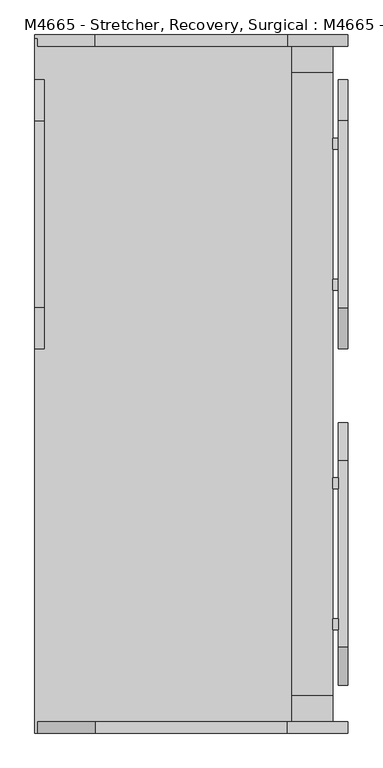
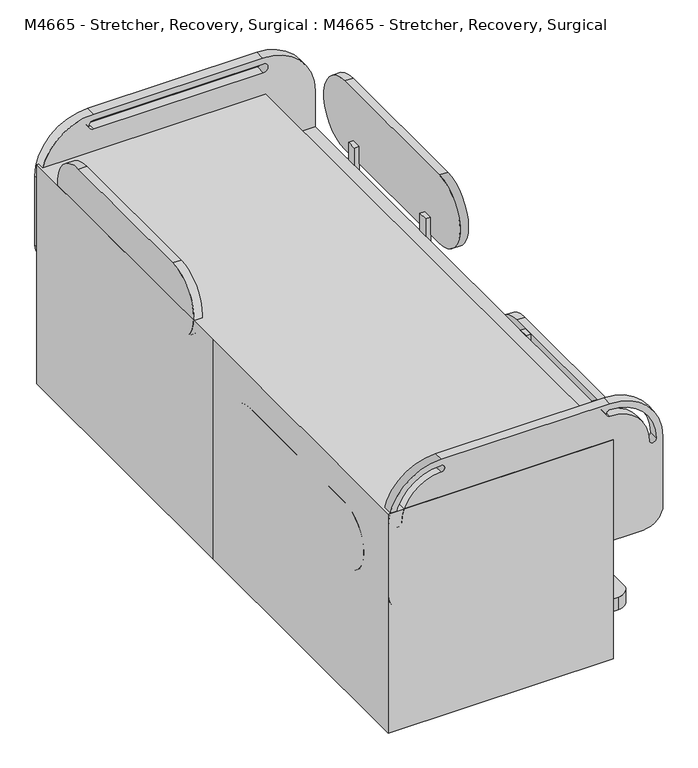
"""IFC4 building model written with IfcOpenShell, lengths in millimetres: proxy geometry, M4665 - Stretcher, Recovery, Surgical : M4665 - Stretcher, Recovery, Surgical."""

import ifcopenshell
import ifcopenshell.guid

model = None  # the IFC model being written
_history = None  # IfcOwnerHistory: only IFC2X3 demands one
_inside = {}  # id of a spatial element -> (the spatial element, [elements in it])
_under = {}  # id of a project, library or spatial element -> (it, [spatial elements below it])
_declared = {}  # id of a project -> (the project, [libraries it declares])
_typed = {}  # id of a type object -> (the type object, [elements of that type])
_made_of = {}  # id of a material, layer set ... -> (it, [elements and type objects made of it])


def new_model(schema):
    """Start an empty IFC model of exactly this schema.

    Asked for "IFC4X3", IfcOpenShell would pick the latest addendum, in which some entities
    have other attributes; the version numbers below select the first issue.
    IFC2X3 requires an IfcOwnerHistory on every rooted entity: one is made here for all.
    """
    global model, _history
    if schema == "IFC4X3":
        model = ifcopenshell.file(schema_version=(4, 3, 0, 0))
    else:
        model = ifcopenshell.file(schema=schema)
    _inside.clear()
    _under.clear()
    _declared.clear()
    _typed.clear()
    _made_of.clear()
    _history = None
    if model.schema == "IFC2X3":
        org = make("IfcOrganization", Name="unknown")
        user = make(
            "IfcPersonAndOrganization",
            ThePerson=make("IfcPerson", FamilyName="unknown"),
            TheOrganization=org,
        )
        app = make(
            "IfcApplication",
            ApplicationDeveloper=org,
            Version="unknown",
            ApplicationFullName="unknown",
            ApplicationIdentifier="unknown",
        )
        _history = make(
            "IfcOwnerHistory",
            OwningUser=user,
            OwningApplication=app,
            ChangeAction="ADDED",
            CreationDate=0,
        )
    return model


def make(cls, **values):
    """One entity of the class cls with the attributes given. An attribute that is None is left unset."""
    return model.create_entity(
        cls, **{name: value for name, value in values.items() if value is not None}
    )


def rooted(cls, **values):
    """An entity with a GlobalId (a new one), such as an element, a storey or a relation."""
    return make(cls, GlobalId=ifcopenshell.guid.new(), OwnerHistory=_history, **values)


def si_unit(unit_type, name, prefix=None):
    """IfcSIUnit, for example si_unit("LENGTHUNIT", "METRE", prefix="MILLI")."""
    return make("IfcSIUnit", UnitType=unit_type, Prefix=prefix, Name=name)


def assignment(units):
    """IfcUnitAssignment: the units of a project."""
    return None if units is None else make("IfcUnitAssignment", Units=units)


def point(xyz):
    """IfcCartesianPoint."""
    return None if xyz is None else make("IfcCartesianPoint", Coordinates=xyz)


def direction(xyz):
    """IfcDirection."""
    return None if xyz is None else make("IfcDirection", DirectionRatios=xyz)


def frame(location, z_axis=None, x_axis=None):
    """IfcAxis2Placement3D, a coordinate frame: its origin and axes. An axis left out is left unset."""
    return make(
        "IfcAxis2Placement3D",
        Location=point(location),
        Axis=direction(z_axis),
        RefDirection=direction(x_axis),
    )


def frame_2d(location, x_axis=None):
    """IfcAxis2Placement2D, a coordinate frame in the plane: its origin and x axis."""
    return make(
        "IfcAxis2Placement2D", Location=point(location), RefDirection=direction(x_axis)
    )


def origin():
    """The frame at (0, 0, 0) with its axes left unset."""
    return frame((0.0, 0.0, 0.0))


def place(relative_to, where):
    """IfcLocalPlacement: puts the frame where relative to a parent placement (None: the world)."""
    return make(
        "IfcLocalPlacement", PlacementRelTo=relative_to, RelativePlacement=where
    )


def context(
    kind, dimensions, precision=None, world=None, true_north=None, identifier=None
):
    """IfcGeometricRepresentationContext, for example the 3D "Model" context."""
    return make(
        "IfcGeometricRepresentationContext",
        ContextIdentifier=identifier,
        ContextType=kind,
        CoordinateSpaceDimension=dimensions,
        Precision=precision,
        WorldCoordinateSystem=world,
        TrueNorth=true_north,
    )


def project(units=None, contexts=None):
    """IfcProject with its units and contexts."""
    return rooted(
        "IfcProject",
        Name="project",
        RepresentationContexts=contexts,
        UnitsInContext=assignment(units),
    )


def spatial(cls, under=None, at=None, **own):
    """A site, building, storey or space (cls), placed at a placement, below another one or the project."""
    s = rooted(cls, ObjectPlacement=at, **own)
    if under is not None:
        _under.setdefault(under.id(), (under, []))[1].append(s)
    return s


def polyline(points):
    """IfcPolyline through the points."""
    return make("IfcPolyline", Points=[point(p) for p in points])


def circle_curve(where, radius):
    """IfcCircle in the frame where."""
    return make("IfcCircle", Position=where, Radius=radius)


def trimmed(basis, trim1, trim2, sense, master):
    """IfcTrimmedCurve: the piece of a basis curve between two trims."""
    return make(
        "IfcTrimmedCurve",
        BasisCurve=basis,
        Trim1=trim1,
        Trim2=trim2,
        SenseAgreement=sense,
        MasterRepresentation=master,
    )


def segment(curve, same_sense, transition):
    """IfcCompositeCurveSegment."""
    return make(
        "IfcCompositeCurveSegment",
        Transition=transition,
        SameSense=same_sense,
        ParentCurve=curve,
    )


def composite_curve(segments, self_intersect=None):
    """IfcCompositeCurve: segments joined end to end."""
    return make("IfcCompositeCurve", Segments=segments, SelfIntersect=self_intersect)


def outline(outer, holes=None, kind="AREA"):
    """IfcArbitraryClosedProfileDef: a profile drawn as a closed curve; with holes, ...WithVoids."""
    if holes is None:
        return make("IfcArbitraryClosedProfileDef", ProfileType=kind, OuterCurve=outer)
    return make(
        "IfcArbitraryProfileDefWithVoids",
        ProfileType=kind,
        OuterCurve=outer,
        InnerCurves=holes,
    )


def extrude(swept, where, along, depth):
    """IfcExtrudedAreaSolid: the profile swept, set in the frame where, extruded along a direction by depth."""
    return make(
        "IfcExtrudedAreaSolid",
        SweptArea=swept,
        Position=where,
        ExtrudedDirection=direction(along),
        Depth=depth,
    )


def faces_of(points, faces, orient=None, outer=None):
    """IfcFace entities. A face is a list of loops; a loop is a list of indices into points, from 0.

    orient and outer hold one flag for each loop. By default every Orientation is true, the
    first loop of a face is its IfcFaceOuterBound and the others are IfcFaceBound.
    """
    made = []
    for i, loops in enumerate(faces):
        bounds = []
        for j, loop in enumerate(loops):
            is_outer = j == 0 if outer is None else outer[i][j]
            bounds.append(
                make(
                    "IfcFaceOuterBound" if is_outer else "IfcFaceBound",
                    Bound=make("IfcPolyLoop", Polygon=[points[k] for k in loop]),
                    Orientation=True if orient is None else orient[i][j],
                )
            )
        made.append(make("IfcFace", Bounds=bounds))
    return made


def faceted_brep(points, faces, orient=None, outer=None, voids=None):
    """IfcFacetedBrep: a solid bounded by flat faces; with voids (closed shells), ...WithVoids."""
    shared = [point(p) for p in points]
    hull = make("IfcClosedShell", CfsFaces=faces_of(shared, faces, orient, outer))
    if voids is None:
        return make("IfcFacetedBrep", Outer=hull)
    return make(
        "IfcFacetedBrepWithVoids",
        Outer=hull,
        Voids=[
            make(cls, CfsFaces=faces_of(shared, fs, o, b)) for cls, fs, o, b in voids
        ],
    )


def shape(context_of_items, identifier, shape_type, items):
    """IfcShapeRepresentation: the items that make up one representation, for example the "Body"."""
    return make(
        "IfcShapeRepresentation",
        ContextOfItems=context_of_items,
        RepresentationIdentifier=identifier,
        RepresentationType=shape_type,
        Items=items,
    )


def source(mapping_origin, context_of_items, identifier, shape_type, items):
    """IfcRepresentationMap: a shape defined once, which mapped items show again and again."""
    return make(
        "IfcRepresentationMap",
        MappingOrigin=mapping_origin,
        MappedRepresentation=shape(context_of_items, identifier, shape_type, items),
    )


def transform(
    local_origin,
    x_axis=None,
    y_axis=None,
    z_axis=None,
    scale=None,
    scale2=None,
    scale3=None,
    uniform=True,
):
    """IfcCartesianTransformationOperator3D, or its non-uniform kind. x_axis, y_axis, z_axis: its Axis1, 2, 3."""
    if uniform:
        return make(
            "IfcCartesianTransformationOperator3D",
            Axis1=direction(x_axis),
            Axis2=direction(y_axis),
            LocalOrigin=point(local_origin),
            Scale=scale,
            Axis3=direction(z_axis),
        )
    return make(
        "IfcCartesianTransformationOperator3DnonUniform",
        Axis1=direction(x_axis),
        Axis2=direction(y_axis),
        LocalOrigin=point(local_origin),
        Scale=scale,
        Axis3=direction(z_axis),
        Scale2=scale2,
        Scale3=scale3,
    )


def mapped(mapping_source, mapping_target):
    """IfcMappedItem: shows the shape of a source again, moved by a transform."""
    return make(
        "IfcMappedItem", MappingSource=mapping_source, MappingTarget=mapping_target
    )


def made_of(thing, what):
    """Note that an element or type object is made of a material, layer set ...; save() writes the relation."""
    if what is not None:
        _made_of.setdefault(what.id(), (what, []))[1].append(thing)
    return thing


def element(
    cls,
    number,
    at=None,
    inside=None,
    cuts=None,
    type_object=None,
    material=None,
    context=None,
    identifier="Body",
    shape_type=None,
    held_by="IfcProductDefinitionShape",
    body=None,
    shapes=None,
    **own,
):
    """One element of the class cls, such as IfcWall. Its Tag is "e" and its number.

    at: its placement. inside: the storey or other place that contains it. cuts: it is an
    opening in that element (IfcRelVoidsElement). A single representation is given by context,
    identifier, shape_type and body (its items); several are given by shapes. held_by: the class
    of the entity that holds the representations. save() writes the other relations.
    """
    e = rooted(cls, Tag="e%d" % number, ObjectPlacement=at, **own)
    if body is not None:
        shapes = [shape(context, identifier, shape_type, body)]
    if shapes is not None:
        e.Representation = make(held_by, Representations=shapes)
    if inside is not None:
        _inside.setdefault(inside.id(), (inside, []))[1].append(e)
    if cuts is not None:
        rooted(
            "IfcRelVoidsElement", RelatingBuildingElement=cuts, RelatedOpeningElement=e
        )
    if type_object is not None:
        _typed.setdefault(type_object.id(), (type_object, []))[1].append(e)
    return made_of(e, material)


def aggregate(whole, parts):
    """IfcRelAggregates: a whole, such as a stair, and the parts it consists of."""
    return rooted("IfcRelAggregates", RelatingObject=whole, RelatedObjects=parts)


def save(model, path):
    """Write the relations noted so far, then the file.

    IfcRelAggregates (storeys below a building ...), IfcRelContainedInSpatialStructure (elements
    in a storey), IfcRelDefinesByType, IfcRelAssociatesMaterial and IfcRelDeclares: one each for
    every whole, place, type object, material and project.
    """
    for whole, parts in _under.values():
        aggregate(whole, parts)
    for where, things in _inside.values():
        rooted(
            "IfcRelContainedInSpatialStructure",
            RelatedElements=things,
            RelatingStructure=where,
        )
    for kind, things in _typed.values():
        rooted("IfcRelDefinesByType", RelatedObjects=things, RelatingType=kind)
    for what, things in _made_of.values():
        rooted("IfcRelAssociatesMaterial", RelatedObjects=things, RelatingMaterial=what)
    for by, libraries in _declared.values():
        rooted("IfcRelDeclares", RelatingContext=by, RelatedDefinitions=libraries)
    model.write(path)


def plane_surface(at):
    """IfcPlane: the flat surface through the origin of the frame at, square to its z axis."""
    return make("IfcPlane", Position=at)


def cylinder_surface(at, radius):
    """IfcCylindricalSurface: all points at the distance radius from the z axis of the frame at."""
    return make("IfcCylindricalSurface", Position=at, Radius=radius)


def revolved_surface(curve, axis_point, axis_direction):
    """IfcSurfaceOfRevolution: the curve turned about the line through axis_point along axis_direction."""
    return make(
        "IfcSurfaceOfRevolution",
        SweptCurve=make("IfcArbitraryOpenProfileDef", ProfileType="CURVE", Curve=curve),
        AxisPosition=make("IfcAxis1Placement", Location=point(axis_point), Axis=direction(axis_direction)),
    )


def advanced_brep(points, edges, surfaces, faces):
    """IfcAdvancedBrep: a solid bounded by faces that lie on surfaces and meet in shared edges.

    An edge is (start, end): straight between two places in points (the first is 0);
    or (start, end, curve); or (start, end, curve, False) where it runs against its curve.
    A face is (place in surfaces, loops), or (place, loops, False) where it looks against
    its surface's normal. A loop lists edges by number (the first is 1), with a minus sign
    where the edge is run from its end to its start. The first loop is the outer one.
    """
    corners = [point(p) for p in points]
    vertices = [make("IfcVertexPoint", VertexGeometry=c) for c in corners]
    made = []
    for start, end, *more in edges:
        made.append(
            make(
                "IfcEdgeCurve",
                EdgeStart=vertices[start],
                EdgeEnd=vertices[end],
                EdgeGeometry=more[0] if more else make("IfcPolyline", Points=[corners[start], corners[end]]),
                SameSense=more[1] if len(more) > 1 else True,
            )
        )
    hull = []
    for where, loops, *sense in faces:
        bounds = []
        for j, loop in enumerate(loops):
            ring = [make("IfcOrientedEdge", EdgeElement=made[abs(k) - 1], Orientation=k > 0) for k in loop]
            bounds.append(
                make(
                    "IfcFaceOuterBound" if j == 0 else "IfcFaceBound",
                    Bound=make("IfcEdgeLoop", EdgeList=ring),
                    Orientation=True,
                )
            )
        hull.append(make("IfcAdvancedFace", Bounds=bounds, FaceSurface=surfaces[where], SameSense=sense[0] if sense else True))
    return make("IfcAdvancedBrep", Outer=make("IfcClosedShell", CfsFaces=hull))


def m4665_stretcher_recovery_surgical_m4665_stretcher_recovery_9e5d2991(model_context):
    return source(origin(), model_context, "Body", "SolidModel", [
        extrude(outline(composite_curve([segment(trimmed(circle_curve(frame_2d((977.7599321, 51.5042315)), 51.5042315), [point((926.2557006, 51.5042315))], [point((1029.2641636, 51.5042315))], False, "CARTESIAN"), True, "CONTINUOUS"), segment(trimmed(circle_curve(frame_2d((977.7599321, 51.5042315)), 51.5042315), [point((1029.2641636, 51.5042315))], [point((926.2557006, 51.5042315))], False, "CARTESIAN"), True, "CONTINUOUS")], self_intersect=False)), frame((-292.1, 0.0, 0.0), z_axis=(1.0, 0.0, 0.0), x_axis=(0.0, 1.0, 0.0)), (0.0, 0.0, 1.0), 25.4),
        extrude(outline(composite_curve([segment(trimmed(circle_curve(frame_2d((977.7599321, 51.5042315)), 51.5042315), [point((926.2557006, 51.5042315))], [point((1029.2641636, 51.5042315))], False, "CARTESIAN"), True, "CONTINUOUS"), segment(trimmed(circle_curve(frame_2d((977.7599321, 51.5042315)), 51.5042315), [point((1029.2641636, 51.5042315))], [point((926.2557006, 51.5042315))], False, "CARTESIAN"), True, "CONTINUOUS")], self_intersect=False)), frame((457.2, 0.0, 0.0), z_axis=(1.0, 0.0, 0.0), x_axis=(0.0, 1.0, 0.0)), (0.0, 0.0, 1.0), 25.4),
        extrude(outline(composite_curve([segment(trimmed(circle_curve(frame_2d((-965.0599321, 51.5042315)), 51.5042315), [point((-913.5557006, 51.5042315))], [point((-1016.5641636, 51.5042315))], False, "CARTESIAN"), True, "CONTINUOUS"), segment(trimmed(circle_curve(frame_2d((-965.0599321, 51.5042315)), 51.5042315), [point((-1016.5641636, 51.5042315))], [point((-913.5557006, 51.5042315))], False, "CARTESIAN"), True, "CONTINUOUS")], self_intersect=False)), frame((457.2, 0.0, 0.0), z_axis=(1.0, 0.0, 0.0), x_axis=(0.0, 1.0, 0.0)), (0.0, 0.0, 1.0), 25.4),
        advanced_brep(
        [(450.85, 990.3863453, 60.4258647), (450.85, 985.39125, 48.3666377), (450.85, 966.5580857, 50.8460708), (450.85, 966.5580857, 108.9715457), (450.85, 976.2356274, 130.175), (450.85, 1006.5868486, 130.175), (450.85, 1014.4209258, 118.4504749), (488.95, 990.3863453, 60.4258647), (488.95, 1014.4209258, 118.4504749), (488.95, 1006.5868486, 130.175), (488.95, 976.2356274, 130.175), (488.95, 966.5580857, 108.9715457), (488.95, 966.5580857, 50.8460708), (488.95, 985.39125, 48.3666377), (457.0636195, 1014.4209258, 118.4504749), (457.0636195, 990.3863453, 60.4258647), (482.4636195, 990.3863453, 60.4258647), (482.4636195, 1014.4209258, 118.4504749), (482.4636195, 1014.7946321, 123.825), (457.0636195, 1014.7946321, 123.825), (457.0636195, 966.5580857, 108.9715457), (457.0636195, 973.337402, 123.825), (482.4636195, 973.337402, 123.825), (482.4636195, 966.5580857, 108.9715457), (457.0636195, 966.5580857, 50.8460708), (482.4636195, 966.5580857, 50.8460708), (457.0636195, 985.39125, 48.3666377), (482.4636195, 985.39125, 48.3666377)],
        [
            (0, 1),
            (1, 2, circle_curve(frame((450.85, 976.1378796, 50.8460708), z_axis=(-1.0, 0.0, 0.0), x_axis=(0.0, -1.0, 0.0)), 9.5797939)),
            (2, 3),
            (3, 4),
            (4, 5),
            (5, 6, circle_curve(frame((450.85, 1006.5868486, 121.6954559), z_axis=(-1.0, 0.0, 0.0), x_axis=(0.0, -1.0, 0.0)), 8.4795441)),
            (6, 0),
            (7, 8),
            (8, 9, circle_curve(frame((488.95, 1006.5868486, 121.6954559), z_axis=(1.0, 0.0, 0.0), x_axis=(0.0, -1.0, 0.0)), 8.4795441)),
            (9, 10),
            (10, 11),
            (11, 12),
            (12, 13, circle_curve(frame((488.95, 976.1378796, 50.8460708), z_axis=(1.0, 0.0, 0.0), x_axis=(0.0, -1.0, 0.0)), 9.5797939)),
            (13, 7),
            (6, 14),
            (14, 15),
            (15, 0),
            (7, 16),
            (16, 17),
            (17, 8),
            (5, 9),
            (17, 18, circle_curve(frame((482.4636195, 1006.5868486, 121.6954559), z_axis=(1.0, 0.0, 0.0), x_axis=(0.0, -1.0, 0.0)), 8.4795441)),
            (18, 19),
            (19, 14, circle_curve(frame((457.0636195, 1006.5868486, 121.6954559), z_axis=(-1.0, 0.0, 0.0), x_axis=(0.0, -1.0, 0.0)), 8.4795441)),
            (4, 10),
            (3, 20),
            (20, 21),
            (21, 22),
            (22, 23),
            (23, 11),
            (2, 24),
            (24, 20),
            (23, 25),
            (25, 12),
            (1, 26),
            (26, 24, circle_curve(frame((457.0636195, 976.1378796, 50.8460708), z_axis=(-1.0, 0.0, 0.0), x_axis=(0.0, -1.0, 0.0)), 9.5797939)),
            (25, 27, circle_curve(frame((482.4636195, 976.1378796, 50.8460708), z_axis=(1.0, 0.0, 0.0), x_axis=(0.0, -1.0, 0.0)), 9.5797939)),
            (27, 13),
            (15, 26),
            (27, 16),
            (18, 22),
            (21, 19),
        ],
        [
            plane_surface(frame((450.85, 990.3863453, 60.4258647), z_axis=(-1.0, 0.0, 0.0), x_axis=(0.0, -0.3826834323651177, -0.9238795325112752))),
            plane_surface(frame((488.95, 990.3863453, 60.4258647), z_axis=(1.0, 0.0, 0.0), x_axis=(0.0, 0.3826834323651177, 0.9238795325112752))),
            plane_surface(frame((450.85, 1014.4209258, 118.4504749), z_axis=(0.0, 0.9238795325112839, -0.38268343236509705), x_axis=(1.0, 0.0, 0.0))),
            cylinder_surface(frame((488.95, 1006.5868486, 121.6954559), z_axis=(-1.0, 0.0, 0.0), x_axis=(0.0, -1.0, 0.0)), 8.4795441),
            plane_surface(frame((450.85, 976.2356274, 130.175), z_axis=(0.0, 0.0, 1.0), x_axis=(1.0, 0.0, 0.0))),
            plane_surface(frame((450.85, 966.5580857, 108.9715457), z_axis=(0.0, -0.9097252183510659, 0.4152108224698697), x_axis=(1.0, 0.0, 0.0))),
            plane_surface(frame((450.85, 966.5580857, 50.8460708), z_axis=(0.0, -1.0, 0.0), x_axis=(1.0, 0.0, 0.0))),
            cylinder_surface(frame((488.95, 976.1378796, 50.8460708), z_axis=(-1.0, 0.0, 0.0), x_axis=(0.0, -1.0, 0.0)), 9.5797939),
            plane_surface(frame((450.85, 990.3863453, 60.4258647), z_axis=(0.0, 0.9238795325112752, -0.3826834323651177), x_axis=(1.0, 0.0, 0.0))),
            plane_surface(frame((482.4636195, 889.3256309, 123.825), z_axis=(0.0, 0.0, -1.0), x_axis=(0.0, 1.0, 0.0))),
            plane_surface(frame((482.4636195, 889.3256309, 0.0), z_axis=(-1.0, 0.0, 0.0), x_axis=(0.0, 1.0, 0.0))),
            plane_surface(frame((457.0636195, 889.3256309, 123.825), z_axis=(1.0, 0.0, 0.0), x_axis=(0.0, 1.0, 0.0))),
        ],
        [
            (0, [[1, 2, 3, 4, 5, 6, 7]]),
            (1, [[8, 9, 10, 11, 12, 13, 14]]),
            (2, [[-7, 15, 16, 17]]),
            (2, [[-8, 18, 19, 20]]),
            (3, [[-6, 21, -9, -20, 22, 23, 24, -15]]),
            (4, [[-5, 25, -10, -21]]),
            (5, [[-4, 26, 27, 28, 29, 30, -11, -25]]),
            (6, [[-3, 31, 32, -26]]),
            (6, [[-12, -30, 33, 34]]),
            (7, [[-2, 35, 36, -31]]),
            (7, [[-13, -34, 37, 38]]),
            (8, [[-1, -17, 39, -35]]),
            (8, [[-14, -38, 40, -18]]),
            (9, [[41, -28, 42, -23]]),
            (10, [[-41, -22, -19, -40, -37, -33, -29]]),
            (11, [[-42, -27, -32, -36, -39, -16, -24]]),
        ],
    ),
        advanced_brep(
        [(-266.5636195, 973.337402, 123.825), (-266.5636195, 1014.7946321, 123.825), (-266.5636195, 1014.4209258, 118.4504749), (-266.5636195, 990.3863453, 60.4258647), (-266.5636195, 985.39125, 48.3666377), (-266.5636195, 966.5580857, 50.8460708), (-266.5636195, 966.5580857, 108.9715457), (-291.9636195, 1014.7946321, 123.825), (-291.9636195, 973.337402, 123.825), (-291.9636195, 966.5580857, 108.9715457), (-291.9636195, 966.5580857, 50.8460708), (-291.9636195, 985.39125, 48.3666377), (-291.9636195, 990.3863453, 60.4258647), (-291.9636195, 1014.4209258, 118.4504749), (-260.35, 990.3863453, 60.4258647), (-260.35, 1014.4209258, 118.4504749), (-260.35, 1006.5868486, 130.175), (-260.35, 976.2356274, 130.175), (-260.35, 966.5580857, 108.9715457), (-260.35, 966.5580857, 50.8460708), (-260.35, 985.39125, 48.3666377), (-298.45, 990.3863453, 60.4258647), (-298.45, 985.39125, 48.3666377), (-298.45, 966.5580857, 50.8460708), (-298.45, 966.5580857, 108.9715457), (-298.45, 976.2356274, 130.175), (-298.45, 1006.5868486, 130.175), (-298.45, 1014.4209258, 118.4504749)],
        [
            (0, 1),
            (1, 2, circle_curve(frame((-266.5636195, 1006.5868486, 121.6954559), z_axis=(-1.0, 0.0, 0.0), x_axis=(0.0, -1.0, 0.0)), 8.4795441)),
            (2, 3),
            (3, 4),
            (4, 5, circle_curve(frame((-266.5636195, 976.1378796, 50.8460708), z_axis=(-1.0, 0.0, 0.0), x_axis=(0.0, -1.0, 0.0)), 9.5797939)),
            (5, 6),
            (6, 0),
            (7, 8),
            (8, 9),
            (9, 10),
            (10, 11, circle_curve(frame((-291.9636195, 976.1378796, 50.8460708), z_axis=(1.0, 0.0, 0.0), x_axis=(0.0, -1.0, 0.0)), 9.5797939)),
            (11, 12),
            (12, 13),
            (13, 7, circle_curve(frame((-291.9636195, 1006.5868486, 121.6954559), z_axis=(1.0, 0.0, 0.0), x_axis=(0.0, -1.0, 0.0)), 8.4795441)),
            (7, 1),
            (0, 8),
            (14, 15),
            (15, 16, circle_curve(frame((-260.35, 1006.5868486, 121.6954559), z_axis=(1.0, 0.0, 0.0), x_axis=(0.0, -1.0, 0.0)), 8.4795441)),
            (16, 17),
            (17, 18),
            (18, 19),
            (19, 20, circle_curve(frame((-260.35, 976.1378796, 50.8460708), z_axis=(1.0, 0.0, 0.0), x_axis=(0.0, -1.0, 0.0)), 9.5797939)),
            (20, 14),
            (21, 22),
            (22, 23, circle_curve(frame((-298.45, 976.1378796, 50.8460708), z_axis=(-1.0, 0.0, 0.0), x_axis=(0.0, -1.0, 0.0)), 9.5797939)),
            (23, 24),
            (24, 25),
            (25, 26),
            (26, 27, circle_curve(frame((-298.45, 1006.5868486, 121.6954559), z_axis=(-1.0, 0.0, 0.0), x_axis=(0.0, -1.0, 0.0)), 8.4795441)),
            (27, 21),
            (20, 4),
            (3, 14),
            (21, 12),
            (11, 22),
            (19, 5),
            (10, 23),
            (18, 6),
            (9, 24),
            (17, 25),
            (16, 26),
            (15, 2),
            (13, 27),
        ],
        [
            plane_surface(frame((-266.5636195, 889.3256309, 0.0), z_axis=(-1.0, 0.0, 0.0), x_axis=(0.0, 1.0, 0.0))),
            plane_surface(frame((-291.9636195, 889.3256309, 123.825), z_axis=(1.0, 0.0, 0.0), x_axis=(0.0, 1.0, 0.0))),
            plane_surface(frame((-266.5636195, 889.3256309, 123.825), z_axis=(0.0, 0.0, -1.0), x_axis=(0.0, 1.0, 0.0))),
            plane_surface(frame((-260.35, 1010.4946248, 108.9715457), z_axis=(1.0000000000000002, 0.0, 0.0), x_axis=(0.0, 0.38268343236509705, 0.9238795325112839))),
            plane_surface(frame((-298.45, 1010.4946248, 108.9715457), z_axis=(-1.0000000000000002, 0.0, 0.0), x_axis=(0.0, -0.38268343236509705, -0.9238795325112839))),
            plane_surface(frame((-260.35, 985.39125, 48.3666377), z_axis=(0.0, 0.9238795325112752, -0.3826834323651177), x_axis=(-1.0, 0.0, 0.0))),
            cylinder_surface(frame((-298.45, 976.1378796, 50.8460708), z_axis=(1.0, 0.0, 0.0), x_axis=(0.0, -1.0, 0.0)), 9.5797939),
            plane_surface(frame((-260.35, 966.5580857, 108.9715457), z_axis=(0.0, -1.0, 0.0), x_axis=(-1.0, 0.0, 0.0))),
            plane_surface(frame((-260.35, 976.2356274, 130.175), z_axis=(0.0, -0.9097252183510659, 0.4152108224698697), x_axis=(-1.0, 0.0, 0.0))),
            plane_surface(frame((-260.35, 1006.5868486, 130.175), z_axis=(0.0, 0.0, 1.0), x_axis=(-1.0, 0.0, 0.0))),
            cylinder_surface(frame((-298.45, 1006.5868486, 121.6954559), z_axis=(1.0, 0.0, 0.0), x_axis=(0.0, -1.0, 0.0)), 8.4795441),
            plane_surface(frame((-260.35, 990.3863453, 60.4258647), z_axis=(0.0, 0.9238795325112839, -0.38268343236509705), x_axis=(-1.0, 0.0, 0.0))),
        ],
        [
            (0, [[1, 2, 3, 4, 5, 6, 7]]),
            (1, [[8, 9, 10, 11, 12, 13, 14]]),
            (2, [[-8, 15, -1, 16]]),
            (3, [[17, 18, 19, 20, 21, 22, 23]]),
            (4, [[24, 25, 26, 27, 28, 29, 30]]),
            (5, [[-23, 31, -4, 32]]),
            (5, [[-24, 33, -12, 34]]),
            (6, [[-22, 35, -5, -31]]),
            (6, [[-25, -34, -11, 36]]),
            (7, [[-21, 37, -6, -35]]),
            (7, [[-26, -36, -10, 38]]),
            (8, [[-20, 39, -27, -38, -9, -16, -7, -37]]),
            (9, [[-19, 40, -28, -39]]),
            (10, [[-18, 41, -2, -15, -14, 42, -29, -40]]),
            (11, [[-17, -32, -3, -41]]),
            (11, [[-30, -42, -13, -33]]),
        ],
    ),
        advanced_brep(
        [(450.85, -977.6863453, 60.4258647), (450.85, -1001.7209258, 118.4504749), (450.85, -993.8868486, 130.175), (450.85, -963.5356274, 130.175), (450.85, -953.8580857, 108.9715457), (450.85, -953.8580857, 50.8460708), (450.85, -972.69125, 48.3666377), (488.95, -977.6863453, 60.4258647), (488.95, -972.69125, 48.3666377), (488.95, -953.8580857, 50.8460708), (488.95, -953.8580857, 108.9715457), (488.95, -963.5356274, 130.175), (488.95, -993.8868486, 130.175), (488.95, -1001.7209258, 118.4504749), (457.0636195, -972.69125, 48.3666377), (457.0636195, -977.6863453, 60.4258647), (482.4636195, -977.6863453, 60.4258647), (482.4636195, -972.69125, 48.3666377), (457.0636195, -953.8580857, 50.8460708), (482.4636195, -953.8580857, 50.8460708), (457.0636195, -953.8580857, 108.9715457), (482.4636195, -953.8580857, 108.9715457), (482.4636195, -960.637402, 123.825), (457.0636195, -960.637402, 123.825), (457.0636195, -1001.7209258, 118.4504749), (457.0636195, -1002.0946321, 123.825), (482.4636195, -1002.0946321, 123.825), (482.4636195, -1001.7209258, 118.4504749)],
        [
            (0, 1),
            (1, 2, circle_curve(frame((450.85, -993.8868486, 121.6954559), z_axis=(-1.0, 0.0, 0.0), x_axis=(0.0, 1.0, 0.0)), 8.4795441)),
            (2, 3),
            (3, 4),
            (4, 5),
            (5, 6, circle_curve(frame((450.85, -963.4378796, 50.8460708), z_axis=(-1.0, 0.0, 0.0), x_axis=(0.0, 1.0, 0.0)), 9.5797939)),
            (6, 0),
            (7, 8),
            (8, 9, circle_curve(frame((488.95, -963.4378796, 50.8460708), z_axis=(1.0, 0.0, 0.0), x_axis=(0.0, 1.0, 0.0)), 9.5797939)),
            (9, 10),
            (10, 11),
            (11, 12),
            (12, 13, circle_curve(frame((488.95, -993.8868486, 121.6954559), z_axis=(1.0, 0.0, 0.0), x_axis=(0.0, 1.0, 0.0)), 8.4795441)),
            (13, 7),
            (6, 14),
            (14, 15),
            (15, 0),
            (7, 16),
            (16, 17),
            (17, 8),
            (5, 18),
            (18, 14, circle_curve(frame((457.0636195, -963.4378796, 50.8460708), z_axis=(-1.0, 0.0, 0.0), x_axis=(0.0, 1.0, 0.0)), 9.5797939)),
            (17, 19, circle_curve(frame((482.4636195, -963.4378796, 50.8460708), z_axis=(1.0, 0.0, 0.0), x_axis=(0.0, 1.0, 0.0)), 9.5797939)),
            (19, 9),
            (4, 20),
            (20, 18),
            (19, 21),
            (21, 10),
            (3, 11),
            (21, 22),
            (22, 23),
            (23, 20),
            (2, 12),
            (1, 24),
            (24, 25, circle_curve(frame((457.0636195, -993.8868486, 121.6954559), z_axis=(-1.0, 0.0, 0.0), x_axis=(0.0, 1.0, 0.0)), 8.4795441)),
            (25, 26),
            (26, 27, circle_curve(frame((482.4636195, -993.8868486, 121.6954559), z_axis=(1.0, 0.0, 0.0), x_axis=(0.0, 1.0, 0.0)), 8.4795441)),
            (27, 13),
            (15, 24),
            (27, 16),
            (23, 25),
            (26, 22),
        ],
        [
            plane_surface(frame((450.85, -997.7946248, 108.9715457), z_axis=(-1.0000000000000002, 0.0, 0.0), x_axis=(0.0, -0.38268343236509705, 0.9238795325112839))),
            plane_surface(frame((488.95, -997.7946248, 108.9715457), z_axis=(1.0000000000000002, 0.0, 0.0), x_axis=(0.0, 0.38268343236509705, -0.9238795325112839))),
            plane_surface(frame((450.85, -972.69125, 48.3666377), z_axis=(0.0, -0.9238795325112752, -0.3826834323651177), x_axis=(1.0, 0.0, 0.0))),
            cylinder_surface(frame((488.95, -963.4378796, 50.8460708), z_axis=(-1.0, 0.0, 0.0), x_axis=(0.0, 1.0, 0.0)), 9.5797939),
            plane_surface(frame((450.85, -953.8580857, 108.9715457), z_axis=(0.0, 1.0, 0.0), x_axis=(1.0, 0.0, 0.0))),
            plane_surface(frame((450.85, -963.5356274, 130.175), z_axis=(0.0, 0.9097252183510659, 0.4152108224698697), x_axis=(1.0, 0.0, 0.0))),
            plane_surface(frame((450.85, -993.8868486, 130.175), z_axis=(0.0, 0.0, 1.0), x_axis=(1.0, 0.0, 0.0))),
            cylinder_surface(frame((488.95, -993.8868486, 121.6954559), z_axis=(-1.0, 0.0, 0.0), x_axis=(0.0, 1.0, 0.0)), 8.4795441),
            plane_surface(frame((450.85, -977.6863453, 60.4258647), z_axis=(0.0, -0.9238795325112839, -0.38268343236509705), x_axis=(1.0, 0.0, 0.0))),
            plane_surface(frame((457.0636195, -876.6256309, 0.0), z_axis=(1.0, 0.0, 0.0), x_axis=(0.0, -1.0, 0.0))),
            plane_surface(frame((482.4636195, -876.6256309, 123.825), z_axis=(-1.0, 0.0, 0.0), x_axis=(0.0, -1.0, 0.0))),
            plane_surface(frame((457.0636195, -876.6256309, 123.825), z_axis=(0.0, 0.0, -1.0), x_axis=(0.0, -1.0, 0.0))),
        ],
        [
            (0, [[1, 2, 3, 4, 5, 6, 7]]),
            (1, [[8, 9, 10, 11, 12, 13, 14]]),
            (2, [[-7, 15, 16, 17]]),
            (2, [[-8, 18, 19, 20]]),
            (3, [[-6, 21, 22, -15]]),
            (3, [[-9, -20, 23, 24]]),
            (4, [[-5, 25, 26, -21]]),
            (4, [[-10, -24, 27, 28]]),
            (5, [[-4, 29, -11, -28, 30, 31, 32, -25]]),
            (6, [[-3, 33, -12, -29]]),
            (7, [[-2, 34, 35, 36, 37, 38, -13, -33]]),
            (8, [[-1, -17, 39, -34]]),
            (8, [[-14, -38, 40, -18]]),
            (9, [[41, -35, -39, -16, -22, -26, -32]]),
            (10, [[42, -30, -27, -23, -19, -40, -37]]),
            (11, [[-42, -36, -41, -31]]),
        ],
    ),
        extrude(outline(composite_curve([segment(trimmed(circle_curve(frame_2d((-965.0599321, 51.5042315)), 51.5042315), [point((-913.5557006, 51.5042315))], [point((-1016.5641636, 51.5042315))], False, "CARTESIAN"), True, "CONTINUOUS"), segment(trimmed(circle_curve(frame_2d((-965.0599321, 51.5042315)), 51.5042315), [point((-1016.5641636, 51.5042315))], [point((-913.5557006, 51.5042315))], False, "CARTESIAN"), True, "CONTINUOUS")], self_intersect=False)), frame((-292.1, 0.0, 0.0), z_axis=(1.0, 0.0, 0.0), x_axis=(0.0, 1.0, 0.0)), (0.0, 0.0, 1.0), 25.4),
        faceted_brep([(-431.8, 1168.4, 889.0), (-431.8, 0.0, 889.0), (-431.8, -1168.4, 889.0), (431.8, -1168.4, 889.0), (431.8, 1168.4, 889.0), (-431.8, 1168.4, 0.0), (431.8, 1168.4, 0.0), (431.8, -1168.4, 0.0), (-431.8, -1168.4, 0.0), (-431.8, 0.0, 0.0), (-291.9636195, 889.3256309, 0.0), (-266.5636195, 889.3256309, 0.0), (-266.5636195, 1064.8184213, 0.0), (-291.9636195, 1064.8184213, 0.0), (-266.5636195, 889.3256309, 123.825), (-291.9636195, 889.3256309, 123.825), (-266.5636195, 1064.8184213, 123.825), (-291.9636195, 1064.8184213, 123.825)], [[[0, 1, 2, 3, 4]], [[5, 6, 7, 8, 9], [10, 11, 12, 13]], [[1, 0, 5, 9]], [[2, 1, 9, 8]], [[3, 2, 8, 7]], [[4, 3, 7, 6]], [[0, 4, 6, 5]], [[14, 11, 10, 15]], [[16, 17, 13, 12]], [[11, 14, 16, 12]], [[15, 10, 13, 17]], [[14, 15, 17, 16]]]),
        advanced_brep(
        [(-260.35, -977.6863453, 60.4258647), (-260.35, -972.69125, 48.3666377), (-260.35, -953.8580857, 50.8460708), (-260.35, -953.8580857, 108.9715457), (-260.35, -963.5356274, 130.175), (-260.35, -993.8868486, 130.175), (-260.35, -1001.7209258, 118.4504749), (-298.45, -977.6863453, 60.4258647), (-298.45, -1001.7209258, 118.4504749), (-298.45, -993.8868486, 130.175), (-298.45, -963.5356274, 130.175), (-298.45, -953.8580857, 108.9715457), (-298.45, -953.8580857, 50.8460708), (-298.45, -972.69125, 48.3666377), (-266.5636195, -977.6863453, 60.4258647), (-266.5636195, -972.69125, 48.3666377), (-291.9636195, -972.69125, 48.3666377), (-291.9636195, -977.6863453, 60.4258647), (-266.5636195, -953.8580857, 50.8460708), (-291.9636195, -953.8580857, 50.8460708), (-266.5636195, -953.8580857, 108.9715457), (-291.9636195, -953.8580857, 108.9715457), (-266.5636195, -960.637402, 123.825), (-291.9636195, -960.637402, 123.825), (-291.9636195, -1001.7209258, 118.4504749), (-291.9636195, -1002.0946321, 123.825), (-266.5636195, -1002.0946321, 123.825), (-266.5636195, -1001.7209258, 118.4504749)],
        [
            (0, 1),
            (1, 2, circle_curve(frame((-260.35, -963.4378796, 50.8460708), z_axis=(1.0, 0.0, 0.0), x_axis=(0.0, 1.0, 0.0)), 9.5797939)),
            (2, 3),
            (3, 4),
            (4, 5),
            (5, 6, circle_curve(frame((-260.35, -993.8868486, 121.6954559), z_axis=(1.0, 0.0, 0.0), x_axis=(0.0, 1.0, 0.0)), 8.4795441)),
            (6, 0),
            (7, 8),
            (8, 9, circle_curve(frame((-298.45, -993.8868486, 121.6954559), z_axis=(-1.0, 0.0, 0.0), x_axis=(0.0, 1.0, 0.0)), 8.4795441)),
            (9, 10),
            (10, 11),
            (11, 12),
            (12, 13, circle_curve(frame((-298.45, -963.4378796, 50.8460708), z_axis=(-1.0, 0.0, 0.0), x_axis=(0.0, 1.0, 0.0)), 9.5797939)),
            (13, 7),
            (0, 14),
            (14, 15),
            (15, 1),
            (13, 16),
            (16, 17),
            (17, 7),
            (15, 18, circle_curve(frame((-266.5636195, -963.4378796, 50.8460708), z_axis=(1.0, 0.0, 0.0), x_axis=(0.0, 1.0, 0.0)), 9.5797939)),
            (18, 2),
            (12, 19),
            (19, 16, circle_curve(frame((-291.9636195, -963.4378796, 50.8460708), z_axis=(-1.0, 0.0, 0.0), x_axis=(0.0, 1.0, 0.0)), 9.5797939)),
            (18, 20),
            (20, 3),
            (11, 21),
            (21, 19),
            (20, 22),
            (22, 23),
            (23, 21),
            (10, 4),
            (9, 5),
            (8, 24),
            (24, 25, circle_curve(frame((-291.9636195, -993.8868486, 121.6954559), z_axis=(-1.0, 0.0, 0.0), x_axis=(0.0, 1.0, 0.0)), 8.4795441)),
            (25, 26),
            (26, 27, circle_curve(frame((-266.5636195, -993.8868486, 121.6954559), z_axis=(1.0, 0.0, 0.0), x_axis=(0.0, 1.0, 0.0)), 8.4795441)),
            (27, 6),
            (27, 14),
            (17, 24),
            (26, 22),
            (23, 25),
        ],
        [
            plane_surface(frame((-260.35, -977.6863453, 60.4258647), z_axis=(1.0, 0.0, 0.0), x_axis=(0.0, 0.3826834323651177, -0.9238795325112752))),
            plane_surface(frame((-298.45, -977.6863453, 60.4258647), z_axis=(-1.0, 0.0, 0.0), x_axis=(0.0, -0.3826834323651177, 0.9238795325112752))),
            plane_surface(frame((-260.35, -977.6863453, 60.4258647), z_axis=(0.0, -0.9238795325112752, -0.3826834323651177), x_axis=(-1.0, 0.0, 0.0))),
            cylinder_surface(frame((-298.45, -963.4378796, 50.8460708), z_axis=(1.0, 0.0, 0.0), x_axis=(0.0, 1.0, 0.0)), 9.5797939),
            plane_surface(frame((-260.35, -953.8580857, 50.8460708), z_axis=(0.0, 1.0, 0.0), x_axis=(-1.0, 0.0, 0.0))),
            plane_surface(frame((-260.35, -953.8580857, 108.9715457), z_axis=(0.0, 0.9097252183510659, 0.4152108224698697), x_axis=(-1.0, 0.0, 0.0))),
            plane_surface(frame((-260.35, -963.5356274, 130.175), z_axis=(0.0, 0.0, 1.0), x_axis=(-1.0, 0.0, 0.0))),
            cylinder_surface(frame((-298.45, -993.8868486, 121.6954559), z_axis=(1.0, 0.0, 0.0), x_axis=(0.0, 1.0, 0.0)), 8.4795441),
            plane_surface(frame((-260.35, -1001.7209258, 118.4504749), z_axis=(0.0, -0.9238795325112839, -0.38268343236509705), x_axis=(-1.0, 0.0, 0.0))),
            plane_surface(frame((-266.5636195, -876.6256309, 123.825), z_axis=(-1.0, 0.0, 0.0), x_axis=(0.0, -1.0, 0.0))),
            plane_surface(frame((-291.9636195, -876.6256309, 0.0), z_axis=(1.0, 0.0, 0.0), x_axis=(0.0, -1.0, 0.0))),
            plane_surface(frame((-291.9636195, -876.6256309, 123.825), z_axis=(0.0, 0.0, -1.0), x_axis=(0.0, -1.0, 0.0))),
        ],
        [
            (0, [[1, 2, 3, 4, 5, 6, 7]]),
            (1, [[8, 9, 10, 11, 12, 13, 14]]),
            (2, [[-1, 15, 16, 17]]),
            (2, [[-14, 18, 19, 20]]),
            (3, [[-2, -17, 21, 22]]),
            (3, [[-13, 23, 24, -18]]),
            (4, [[-3, -22, 25, 26]]),
            (4, [[-12, 27, 28, -23]]),
            (5, [[-4, -26, 29, 30, 31, -27, -11, 32]]),
            (6, [[-5, -32, -10, 33]]),
            (7, [[-6, -33, -9, 34, 35, 36, 37, 38]]),
            (8, [[-7, -38, 39, -15]]),
            (8, [[-8, -20, 40, -34]]),
            (9, [[41, -29, -25, -21, -16, -39, -37]]),
            (10, [[42, -35, -40, -19, -24, -28, -31]]),
            (11, [[-41, -36, -42, -30]]),
        ],
    ),
        extrude(outline(polyline([(260.35, 850.9), (-69.85, 850.9), (-69.85, 1054.1), (260.35, 1054.1), (260.35, 850.9)])), frame((0.0, 0.0, 180.975), z_axis=(0.0, 0.0, 1.0), x_axis=(1.0, 0.0, 0.0)), (0.0, 0.0, 1.0), 325.7374197),
        extrude(outline(polyline([(260.35, -1041.4), (-69.85, -1041.4), (-69.85, -838.2), (260.35, -838.2), (260.35, -1041.4)])), frame((0.0, 0.0, 180.975), z_axis=(0.0, 0.0, 1.0), x_axis=(1.0, 0.0, 0.0)), (0.0, 0.0, 1.0), 325.7374197),
        advanced_brep(
        [(419.1, 1143.0, 1039.6271945), (-228.6, 1143.0, 1039.6271945), (-431.8, 1143.0, 836.4271945), (-431.8, 1143.0, 557.5709378), (-355.6, 1143.0, 481.3709378), (546.1, 1143.0, 481.3709378), (622.3, 1143.0, 557.5709378), (622.3, 1143.0, 836.4271945), (422.9792937, 1143.0, 1014.18421), (423.0083062, 1143.0, 979.3021945), (-228.6, 1143.0, 979.3021945), (-228.6, 1143.0, 1014.2271945), (419.1, 1181.1, 1039.6271945), (622.3, 1181.1, 836.4271945), (622.3, 1181.1, 557.5709378), (546.1, 1181.1, 481.3709378), (-355.6, 1181.1, 481.3709378), (-431.8, 1181.1, 557.5709378), (-431.8, 1181.1, 836.4271945), (-228.6, 1181.1, 1039.6271945), (423.0083062, 1181.1, 979.3021945), (422.9792937, 1181.1, 1014.18421), (-228.6, 1181.1, 1014.2271945), (-228.6, 1181.1, 979.3021945)],
        [
            (0, 1),
            (1, 2, circle_curve(frame((-228.6, 1143.0, 836.4271945), z_axis=(0.0, -1.0, 0.0), x_axis=(-1.0, 0.0, 0.0)), 203.2)),
            (2, 3),
            (3, 4, circle_curve(frame((-355.6, 1143.0, 557.5709378), z_axis=(0.0, -1.0, 0.0), x_axis=(-1.0, 0.0, 0.0)), 76.2)),
            (4, 5),
            (5, 6, circle_curve(frame((546.1, 1143.0, 557.5709378), z_axis=(0.0, -1.0, 0.0), x_axis=(-1.0, 0.0, 0.0)), 76.2)),
            (6, 7),
            (7, 0, circle_curve(frame((419.1, 1143.0, 836.4271945), z_axis=(0.0, -1.0, 0.0), x_axis=(-1.0, 0.0, 0.0)), 203.2)),
            (8, 9, circle_curve(frame((423.0083062, 1143.0, 996.7432143), z_axis=(0.0, 1.0, 0.0), x_axis=(-1.0, 0.0, 0.0)), 17.4410198)),
            (9, 10),
            (10, 11, circle_curve(frame((-228.6, 1143.0, 996.7646945), z_axis=(0.0, 1.0, 0.0), x_axis=(-1.0, 0.0, 0.0)), 17.4625)),
            (11, 8),
            (12, 13, circle_curve(frame((419.1, 1181.1, 836.4271945), z_axis=(0.0, 1.0, 0.0), x_axis=(-1.0, 0.0, 0.0)), 203.2)),
            (13, 14),
            (14, 15, circle_curve(frame((546.1, 1181.1, 557.5709378), z_axis=(0.0, 1.0, 0.0), x_axis=(-1.0, 0.0, 0.0)), 76.2)),
            (15, 16),
            (16, 17, circle_curve(frame((-355.6, 1181.1, 557.5709378), z_axis=(0.0, 1.0, 0.0), x_axis=(-1.0, 0.0, 0.0)), 76.2)),
            (17, 18),
            (18, 19, circle_curve(frame((-228.6, 1181.1, 836.4271945), z_axis=(0.0, 1.0, 0.0), x_axis=(-1.0, 0.0, 0.0)), 203.2)),
            (19, 12),
            (20, 21, circle_curve(frame((423.0083062, 1181.1, 996.7432143), z_axis=(0.0, -1.0, 0.0), x_axis=(-1.0, 0.0, 0.0)), 17.4410198)),
            (21, 22),
            (22, 23, circle_curve(frame((-228.6, 1181.1, 996.7646945), z_axis=(0.0, -1.0, 0.0), x_axis=(-1.0, 0.0, 0.0)), 17.4625)),
            (23, 20),
            (0, 12),
            (19, 1),
            (18, 2),
            (17, 3),
            (16, 4),
            (15, 5),
            (14, 6),
            (13, 7),
            (20, 9),
            (8, 21),
            (23, 10),
            (22, 11),
        ],
        [
            plane_surface(frame((-228.6, 1143.0, 1039.6271945), z_axis=(0.0, -1.0, 0.0), x_axis=(-1.0, 0.0, 0.0))),
            plane_surface(frame((-228.6, 1181.1, 1039.6271945), z_axis=(0.0, 1.0, 0.0), x_axis=(1.0, 0.0, 0.0))),
            plane_surface(frame((419.1, 1143.0, 1039.6271945), z_axis=(0.0, 0.0, 1.0), x_axis=(0.0, 1.0, 0.0))),
            cylinder_surface(frame((-228.6, 1181.1, 836.4271945), z_axis=(0.0, -1.0, 0.0), x_axis=(-1.0, 0.0, 0.0)), 203.2),
            plane_surface(frame((-431.8, 1143.0, 836.4271945), z_axis=(-1.0, 0.0, 0.0), x_axis=(0.0, 1.0, 0.0))),
            cylinder_surface(frame((-355.6, 1181.1, 557.5709378), z_axis=(0.0, -1.0, 0.0), x_axis=(-1.0, 0.0, 0.0)), 76.2),
            plane_surface(frame((-355.6, 1143.0, 481.3709378), z_axis=(0.0, 0.0, -1.0), x_axis=(0.0, 1.0, 0.0))),
            cylinder_surface(frame((546.1, 1181.1, 557.5709378), z_axis=(0.0, -1.0, 0.0), x_axis=(-1.0, 0.0, 0.0)), 76.2),
            plane_surface(frame((622.3, 1143.0, 557.5709378), z_axis=(1.0, 0.0, 0.0), x_axis=(0.0, 1.0, 0.0))),
            cylinder_surface(frame((419.1, 1181.1, 836.4271945), z_axis=(0.0, -1.0, 0.0), x_axis=(-1.0, 0.0, 0.0)), 203.2),
            revolved_surface(polyline([(405.5672864, 1181.1, 996.7432143), (405.5672864, 1143.0, 996.7432143)]), (423.0083062, 1143.0, 996.7432143), (0.0, 1.0, 0.0)),
            plane_surface(frame((423.0083062, 1181.1, 979.3021945), z_axis=(0.0, 0.0, 1.0), x_axis=(0.0, -1.0, 0.0))),
            revolved_surface(polyline([(-246.0625, 1181.1, 996.7646945), (-246.0625, 1143.0, 996.7646945)]), (-228.6, 1143.0, 996.7646945), (0.0, 1.0, 0.0)),
            plane_surface(frame((-228.6, 1181.1, 1014.2271945), z_axis=(0.0, 0.0, -1.0), x_axis=(0.0, -1.0, 0.0))),
        ],
        [
            (0, [[1, 2, 3, 4, 5, 6, 7, 8], [9, 10, 11, 12]]),
            (1, [[13, 14, 15, 16, 17, 18, 19, 20], [21, 22, 23, 24]]),
            (2, [[-1, 25, -20, 26]]),
            (3, [[-2, -26, -19, 27]]),
            (4, [[-3, -27, -18, 28]]),
            (5, [[-4, -28, -17, 29]]),
            (6, [[-5, -29, -16, 30]]),
            (7, [[-6, -30, -15, 31]]),
            (8, [[-7, -31, -14, 32]]),
            (9, [[-8, -32, -13, -25]]),
            (10, [[33, -9, 34, -21]]),
            (11, [[-33, -24, 35, -10]]),
            (12, [[-35, -23, 36, -11]]),
            (13, [[-34, -12, -36, -22]]),
        ],
    ),
        extrude(outline(composite_curve([segment(polyline([(1039.6271945, 419.1), (1039.6271945, -228.6)]), True, "CONTINUOUS"), segment(trimmed(circle_curve(frame_2d((836.4271945, -228.6)), 203.2), [point((1039.6271945, -228.6))], [point((836.4271945, -431.8))], False, "CARTESIAN"), True, "CONTINUOUS"), segment(polyline([(836.4271945, -431.8), (557.5709378, -431.8)]), True, "CONTINUOUS"), segment(trimmed(circle_curve(frame_2d((557.5709378, -355.6)), 76.2), [point((557.5709378, -431.8))], [point((481.3709378, -355.6))], False, "CARTESIAN"), True, "CONTINUOUS"), segment(polyline([(481.3709378, -355.6), (481.3709378, 546.1)]), True, "CONTINUOUS"), segment(trimmed(circle_curve(frame_2d((557.5709378, 546.1)), 76.2), [point((481.3709378, 546.1))], [point((557.5709378, 622.3))], False, "CARTESIAN"), True, "CONTINUOUS"), segment(polyline([(557.5709378, 622.3), (836.4271945, 622.3)]), True, "CONTINUOUS"), segment(trimmed(circle_curve(frame_2d((836.4271945, 419.1)), 203.2), [point((836.4271945, 622.3))], [point((1039.6271945, 419.1))], False, "CARTESIAN"), True, "CONTINUOUS")], self_intersect=False), holes=[composite_curve([segment(trimmed(circle_curve(frame_2d((1001.5271945, -228.6)), 12.7), [point((1014.2271945, -228.6))], [point((988.8271945, -228.6))], True, "CARTESIAN"), True, "CONTINUOUS"), segment(trimmed(circle_curve(frame_2d((836.4271945, -228.6)), 152.4), [point((988.8271945, -228.6))], [point((836.4271945, -381.0))], False, "CARTESIAN"), True, "CONTINUOUS"), segment(trimmed(circle_curve(frame_2d((836.4271945, -393.7)), 12.7), [point((836.4271945, -381.0))], [point((836.4271945, -406.4))], True, "CARTESIAN"), True, "CONTINUOUS"), segment(trimmed(circle_curve(frame_2d((836.4271945, -228.6)), 177.8), [point((836.4271945, -406.4))], [point((1014.2271945, -228.6))], True, "CARTESIAN"), True, "CONTINUOUS")], self_intersect=False), composite_curve([segment(trimmed(circle_curve(frame_2d((836.4271945, 584.2)), 12.7), [point((836.4271945, 596.9))], [point((836.4271945, 571.5))], True, "CARTESIAN"), True, "CONTINUOUS"), segment(trimmed(circle_curve(frame_2d((836.4271945, 419.1)), 152.4), [point((836.4271945, 571.5))], [point((988.8271945, 419.1))], False, "CARTESIAN"), True, "CONTINUOUS"), segment(trimmed(circle_curve(frame_2d((1001.5271945, 419.1)), 12.7), [point((988.8271945, 419.1))], [point((1014.2271945, 419.1))], True, "CARTESIAN"), True, "CONTINUOUS"), segment(trimmed(circle_curve(frame_2d((836.4271945, 419.1)), 177.8), [point((1014.2271945, 419.1))], [point((836.4271945, 596.9))], True, "CARTESIAN"), True, "CONTINUOUS")], self_intersect=False)]), frame((0.0, -1168.4, 0.0), z_axis=(0.0, 1.0, 0.0), x_axis=(0.0, 0.0, 1.0)), (0.0, 0.0, 1.0), 38.1),
        extrude(outline(polyline([(571.4543388, -346.6603976), (571.4543388, -308.5603976), (590.3241731, -308.5603976), (590.3241731, -346.6603976), (571.4543388, -346.6603976)])), frame((0.0, 0.0, 506.7124197), z_axis=(0.0, 0.0, 1.0), x_axis=(1.0, 0.0, 0.0)), (0.0, 0.0, 1.0), 255.2875803),
        extrude(outline(polyline([(571.4543388, -821.1211377), (571.4543388, -783.0211377), (590.3241731, -783.0211377), (590.3241731, -821.1211377), (571.4543388, -821.1211377)])), frame((0.0, 0.0, 506.7124197), z_axis=(0.0, 0.0, 1.0), x_axis=(1.0, 0.0, 0.0)), (0.0, 0.0, 1.0), 255.2875803),
        extrude(outline(composite_curve([segment(trimmed(circle_curve(frame_2d((-250.5157677, 634.3562098)), 127.6437902), [point((-250.5157677, 762.0))], [point((-250.5157677, 506.7124197))], False, "CARTESIAN"), True, "CONTINUOUS"), segment(polyline([(-250.5157677, 506.7124197), (-879.1657677, 506.7124197)]), True, "CONTINUOUS"), segment(trimmed(circle_curve(frame_2d((-879.1657677, 634.3562098)), 127.6437902), [point((-879.1657677, 506.7124197))], [point((-879.1657677, 762.0))], False, "CARTESIAN"), True, "CONTINUOUS"), segment(polyline([(-879.1657677, 762.0), (-250.5157677, 762.0)]), True, "CONTINUOUS")], self_intersect=False)), frame((590.3241731, 0.0, 0.0), z_axis=(1.0, 0.0, 0.0), x_axis=(0.0, 1.0, 0.0)), (0.0, 0.0, 1.0), 31.9758269),
        extrude(outline(polyline([(571.4543388, 321.2603976), (571.4543388, 359.3603976), (590.3241731, 359.3603976), (590.3241731, 321.2603976), (571.4543388, 321.2603976)])), frame((0.0, 0.0, 506.7124197), z_axis=(0.0, 0.0, 1.0), x_axis=(1.0, 0.0, 0.0)), (0.0, 0.0, 1.0), 325.1375803),
        extrude(outline(polyline([(571.4543388, 795.7211377), (571.4543388, 833.8211377), (590.3241731, 833.8211377), (590.3241731, 795.7211377), (571.4543388, 795.7211377)])), frame((0.0, 0.0, 506.7124197), z_axis=(0.0, 0.0, 1.0), x_axis=(1.0, 0.0, 0.0)), (0.0, 0.0, 1.0), 325.1375803),
        extrude(outline(composite_curve([segment(polyline([(263.2157677, 1039.6271945), (891.8657677, 1039.6271945)]), True, "CONTINUOUS"), segment(trimmed(circle_curve(frame_2d((891.8657677, 900.8135972)), 138.8135972), [point((891.8657677, 1039.6271945))], [point((891.8657677, 762.0))], False, "CARTESIAN"), True, "CONTINUOUS"), segment(polyline([(891.8657677, 762.0), (263.2157677, 762.0)]), True, "CONTINUOUS"), segment(trimmed(circle_curve(frame_2d((263.2157677, 900.8135972)), 138.8135972), [point((263.2157677, 762.0))], [point((263.2157677, 1039.6271945))], False, "CARTESIAN"), True, "CONTINUOUS")], self_intersect=False)), frame((590.3241731, 0.0, 0.0), z_axis=(1.0, 0.0, 0.0), x_axis=(0.0, 1.0, 0.0)), (0.0, 0.0, 1.0), 31.9758269),
        extrude(outline(polyline([(-381.3704979, -308.5603976), (-381.3704979, -346.6603976), (-399.8241731, -346.6603976), (-399.8241731, -308.5603976), (-381.3704979, -308.5603976)])), frame((0.0, 0.0, 506.7124197), z_axis=(0.0, 0.0, 1.0), x_axis=(1.0, 0.0, 0.0)), (0.0, 0.0, 1.0), 255.2875803),
        extrude(outline(polyline([(-381.3704979, -783.0211377), (-381.3704979, -821.1211377), (-399.8241731, -821.1211377), (-399.8241731, -783.0211377), (-381.3704979, -783.0211377)])), frame((0.0, 0.0, 506.7124197), z_axis=(0.0, 0.0, 1.0), x_axis=(1.0, 0.0, 0.0)), (0.0, 0.0, 1.0), 255.2875803),
        extrude(outline(composite_curve([segment(trimmed(circle_curve(frame_2d((-250.5157677, 634.3562098)), 127.6437902), [point((-250.5157677, 762.0))], [point((-250.5157677, 506.7124197))], False, "CARTESIAN"), True, "CONTINUOUS"), segment(polyline([(-250.5157677, 506.7124197), (-879.1657677, 506.7124197)]), True, "CONTINUOUS"), segment(trimmed(circle_curve(frame_2d((-879.1657677, 634.3562098)), 127.6437902), [point((-879.1657677, 506.7124197))], [point((-879.1657677, 762.0))], False, "CARTESIAN"), True, "CONTINUOUS"), segment(polyline([(-879.1657677, 762.0), (-250.5157677, 762.0)]), True, "CONTINUOUS")], self_intersect=False)), frame((-431.8, 0.0, 0.0), z_axis=(1.0, 0.0, 0.0), x_axis=(0.0, 1.0, 0.0)), (0.0, 0.0, 1.0), 31.9758269),
        extrude(outline(polyline([(-381.3704979, 359.3603976), (-381.3704979, 321.2603976), (-399.8241731, 321.2603976), (-399.8241731, 359.3603976), (-381.3704979, 359.3603976)])), frame((0.0, 0.0, 506.7124197), z_axis=(0.0, 0.0, 1.0), x_axis=(1.0, 0.0, 0.0)), (0.0, 0.0, 1.0), 325.1375803),
        extrude(outline(polyline([(-381.3704979, 833.8211377), (-381.3704979, 795.7211377), (-399.8241731, 795.7211377), (-399.8241731, 833.8211377), (-381.3704979, 833.8211377)])), frame((0.0, 0.0, 506.7124197), z_axis=(0.0, 0.0, 1.0), x_axis=(1.0, 0.0, 0.0)), (0.0, 0.0, 1.0), 325.1375803),
        extrude(outline(composite_curve([segment(polyline([(263.2157677, 1039.6271945), (891.8657677, 1039.6271945)]), True, "CONTINUOUS"), segment(trimmed(circle_curve(frame_2d((891.8657677, 900.8135972)), 138.8135972), [point((891.8657677, 1039.6271945))], [point((891.8657677, 762.0))], False, "CARTESIAN"), True, "CONTINUOUS"), segment(polyline([(891.8657677, 762.0), (263.2157677, 762.0)]), True, "CONTINUOUS"), segment(trimmed(circle_curve(frame_2d((263.2157677, 900.8135972)), 138.8135972), [point((263.2157677, 762.0))], [point((263.2157677, 1039.6271945))], False, "CARTESIAN"), True, "CONTINUOUS")], self_intersect=False)), frame((-431.8, 0.0, 0.0), z_axis=(1.0, 0.0, 0.0), x_axis=(0.0, 1.0, 0.0)), (0.0, 0.0, 1.0), 31.9758269),
        extrude(outline(polyline([(571.4543388, 1054.1), (571.4543388, -1041.4), (-381.3704979, -1041.4), (-381.3704979, 1054.1), (571.4543388, 1054.1)])), frame((0.0, 0.0, 557.6073872), z_axis=(0.0, 0.0, 1.0), x_axis=(1.0, 0.0, 0.0)), (0.0, 0.0, 1.0), 204.3926128),
        extrude(outline(polyline([(571.4543388, 1143.0), (571.4543388, -1130.3), (-381.3704979, -1130.3), (-381.3704979, 1143.0), (571.4543388, 1143.0)])), frame((0.0, 0.0, 506.7124197), z_axis=(0.0, 0.0, 1.0), x_axis=(1.0, 0.0, 0.0)), (0.0, 0.0, 1.0), 50.8949675),
        extrude(outline(composite_curve([segment(trimmed(circle_curve(frame_2d((495.3, 1054.1)), 50.8), [point((495.3, 1104.9))], [point((546.1, 1054.1))], False, "CARTESIAN"), True, "CONTINUOUS"), segment(polyline([(546.1, 1054.1), (546.1, 800.1), (393.7, 800.1), (393.7, -787.4), (546.1, -787.4), (546.1, -1041.4)]), True, "CONTINUOUS"), segment(trimmed(circle_curve(frame_2d((495.3, -1041.4)), 50.8), [point((546.1, -1041.4))], [point((495.3, -1092.2))], False, "CARTESIAN"), True, "CONTINUOUS"), segment(polyline([(495.3, -1092.2), (-304.8, -1092.2)]), True, "CONTINUOUS"), segment(trimmed(circle_curve(frame_2d((-304.8, -1041.4)), 50.8), [point((-304.8, -1092.2))], [point((-355.6, -1041.4))], False, "CARTESIAN"), True, "CONTINUOUS"), segment(polyline([(-355.6, -1041.4), (-355.6, -787.4), (-203.2, -787.4), (-203.2, 800.1), (-355.6, 800.1), (-355.6, 1054.1)]), True, "CONTINUOUS"), segment(trimmed(circle_curve(frame_2d((-304.8, 1054.1)), 50.8), [point((-355.6, 1054.1))], [point((-304.8, 1104.9))], False, "CARTESIAN"), True, "CONTINUOUS"), segment(polyline([(-304.8, 1104.9), (495.3, 1104.9)]), True, "CONTINUOUS")], self_intersect=False)), frame((0.0, 0.0, 130.175), z_axis=(0.0, 0.0, 1.0), x_axis=(1.0, 0.0, 0.0)), (0.0, 0.0, 1.0), 50.8),
    ])


if __name__ == "__main__":
    model = new_model("IFC4")
    model_context = context("Model", 3, world=origin())
    ifc_project = project(units=[si_unit("LENGTHUNIT", "METRE", prefix="MILLI")], contexts=[model_context])
    site = spatial("IfcSite", under=ifc_project)
    building = spatial("IfcBuilding", under=site)
    placement = place(None, origin())
    m4665_stretcher_recovery_surgical_m4665_stretcher_recovery_shape = m4665_stretcher_recovery_surgical_m4665_stretcher_recovery_9e5d2991(model_context)
    element("IfcBuildingElementProxy", 1, Name="M4665 - Stretcher, Recovery, Surgical : M4665 - Stretcher, Recovery, Surgical", ObjectType="M4665 - Stretcher, Recovery, Surgical : M4665 - Stretcher, Recovery, Surgical", at=placement, inside=building, context=model_context, shape_type="MappedRepresentation", body=[
        mapped(m4665_stretcher_recovery_surgical_m4665_stretcher_recovery_shape, transform((0.0, 0.0, 0.0), x_axis=(1.0, 0.0, 0.0), y_axis=(0.0, 1.0, 0.0), z_axis=(0.0, 0.0, 1.0))),
    ])
    save(model, "model.ifc")

# Revit data of these elements
# Project information
#   Room Abbreviation = "RROP2"
#   Room Description = "Recovery Cubicle, Phase II (RROP2)"
#   Sheets - Total = "5"
#   Project Issue Date = "Issue Date"
#   Project Status = "Project Status"
#   Client Name = "Owner"
#   Project Address = "Enter address here"
#   Project Name = "Project Name"
#   Project Number = "Project Number"
#   Publication Date = "30-Jan-15"
# Type "M4665 - Stretcher, Recovery, Surgical : M4665 - Stretcher, Recovery, Surgical"
#   Watts2 = "0"
#   Watts1 = "0"
#   Unit_Issue = "EA"
#   UTIL_6_Misc = "-"
#   UTIL_5_NonMedGas = "-"
#   UTIL_4_MiscGas = "-"
#   UTIL_3_MedGas = "-"
#   UTIL_2_Elec = "-"
#   UTIL_1_WaterDrain = "-"
#   Nomenclature = "Stretcher, Recovery, Surgical"
#   NSN = "6530"
#   Location [instance default] = ""
#   JSN = "M4665"
#   Fund_Source_VA = "-"
#   Fund_Source_Navy = "-"
#   Fund_Source_Army = "-"
#   Fund_Source_AF = "-"
#   ELEC_Volts2 = "0"
#   ELEC_Volts1 = "0"
#   ELEC_Phase2 = "0"
#   ELEC_Phase1 = "0"
#   ELEC_HertzSwitch = "0"
#   ELEC_HertzDependent = "0"
#   ELEC_Hertz = "0"
#   ELEC_Amps2 = "0"
#   ELEC_Amps1 = "0"
#   DetailDescription = "Recovery/surgical stretcher. Strong I-beam construction type unit. The height is adjustable with manual backrest and crank operated knee gatch. Stainless or painted steel top and chassis. Features 8\" or 10\" conductive casters, with lock and brake, folding, tuck-away chrome side-rails and IV stand and a flame retardant antibacterial mattress. Designed for operating room transport or recovery applications."
#   CAT_VA = "C"
#   CAT_Navy = "C"
#   CAT_IHS = "-"
#   CAT_Army = "C"
#   CAT_AF = "C"
#   BTUperhour = "0"
#   width base support = 0' - 0"
#   Weight_IP = 276
#   DIM_Width_IP = 2' - 10"
#   DIM_Height_IP = 2' - 11"
#   DIM_Depth_IP = 7' - 8"
#   mattress [instance default] = none
#   head / foor board [instance default] = none
#   frame [instance default] = none
#   caster material [instance default] = none
# Element 1 (IfcBuildingElementProxy, "M4665 - Stretcher, Recovery, Surgical : M4665 - Stretcher, Recovery, Surgical")
#   Location = "RROP1"
#   Materials on its faces: "EquipSpace"
# Materials
#   "EquipSpace": class "Unassigned", colour RGB 221 217 195, transparency 0.5
